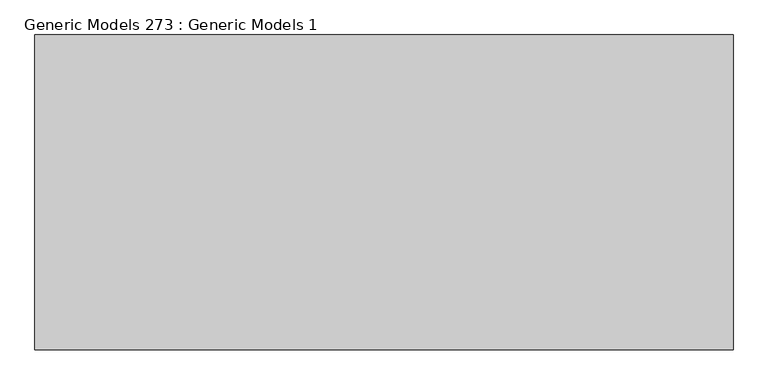
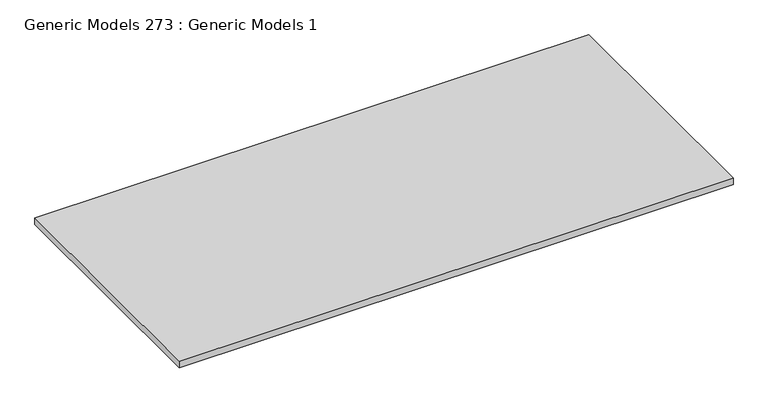
"""IFC4 building model written with IfcOpenShell, lengths in millimetres: proxy geometry, Generic Models 273 : Generic Models 1."""

from ifc_helpers import new_model, si_unit, frame, origin, place, context, project, spatial, polyline, outline, extrude, source, transform, mapped, element, save


def generic_models_273_generic_models_1_8c366405(model_context):
    return source(origin(), model_context, "Body", "SweptSolid", [
        extrude(outline(polyline([(-2005.403384, 1085.2769662), (-484.7895797, 1085.2769662), (-484.7895797, 399.7309662), (-2005.403384, 399.7309662), (-2005.403384, 1085.2769662)])), frame((0.0, 0.0, 126783.846), z_axis=(0.0, 0.0, 1.0), x_axis=(1.0, 0.0, 0.0)), (0.0, 0.0, 1.0), 19.05),
    ])


if __name__ == "__main__":
    model = new_model("IFC4")
    model_context = context("Model", 3, world=origin())
    ifc_project = project(units=[si_unit("LENGTHUNIT", "METRE", prefix="MILLI")], contexts=[model_context])
    site = spatial("IfcSite", under=ifc_project)
    building = spatial("IfcBuilding", under=site)
    placement = place(None, origin())
    generic_models_273_generic_models_1_shape = generic_models_273_generic_models_1_8c366405(model_context)
    element("IfcBuildingElementProxy", 1, Name="Generic Models 273 : Generic Models 1", ObjectType="Generic Models 273 : Generic Models 1", at=placement, inside=building, context=model_context, shape_type="MappedRepresentation", body=[
        mapped(generic_models_273_generic_models_1_shape, transform((0.0, 0.0, 0.0), x_axis=(1.0, 0.0, 0.0), y_axis=(0.0, 1.0, 0.0), z_axis=(0.0, 0.0, 1.0))),
    ])
    save(model, "model.ifc")

# Revit data of these elements
# Element 1 (IfcBuildingElementProxy, "Generic Models 273 : Generic Models 1")
#   Materials on its faces: "_CDX PLYWOOD - SEE STRUCT DWGs"
# Materials
#   "_CDX PLYWOOD - SEE STRUCT DWGs": class "Generic", colour RGB 98 75 74, transparency 0, Cost = 0
